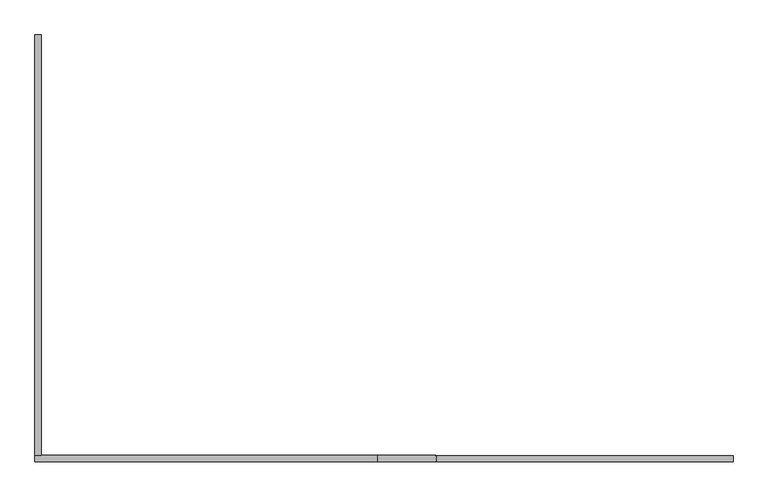
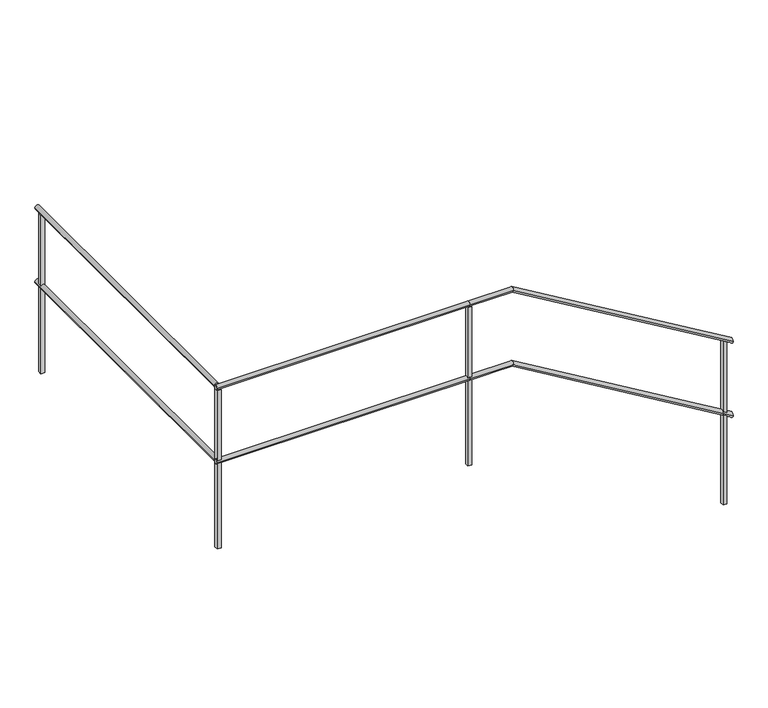
"""IFC4 building model written with IfcOpenShell, lengths in millimetres: railing geometry."""

from ifc_helpers import new_model, si_unit, frame, origin, place, context, project, spatial, polyline, circle_curve, ellipse_curve, outline, extrude, source, transform, mapped, element, save
from ifc_brep_helpers import plane_surface, cylinder_surface, advanced_brep


def railing_f3a6625a(model_context):
    return source(origin(), model_context, "Body", "SolidModel", [
        advanced_brep(
        [(26565.4, 649.5208589, 1734.9618634), (26535.4, 649.5208589, 1734.9618634), (26565.4, -1335.0791411, 1734.9618634), (26535.4, -1335.0791411, 1734.9618634)],
        [
            (0, 1, circle_curve(frame((26550.4, 649.5208589, 1734.9618634), z_axis=(0.0, 1.0, 0.0), x_axis=(-1.0, 0.0, 0.0)), 15.0)),
            (1, 0, circle_curve(frame((26550.4, 649.5208589, 1734.9618634), z_axis=(0.0, 1.0, 0.0), x_axis=(-1.0, 0.0, 0.0)), 15.0)),
            (2, 3, circle_curve(frame((26550.4, -1335.0791411, 1734.9618634), z_axis=(0.0, -1.0, 0.0), x_axis=(-1.0, 0.0, 0.0)), 15.0)),
            (3, 2, circle_curve(frame((26550.4, -1335.0791411, 1734.9618634), z_axis=(0.0, -1.0, 0.0), x_axis=(-1.0, 0.0, 0.0)), 15.0)),
            (0, 2),
            (3, 1),
        ],
        [
            plane_surface(frame((26550.4, 649.5208589, 1749.9618634), z_axis=(0.0, 1.0, 0.0), x_axis=(0.0, 0.0, -1.0))),
            plane_surface(frame((26550.4, -1335.0791411, 1749.9618634), z_axis=(0.0, -1.0, 0.0), x_axis=(0.0, 0.0, -1.0))),
            cylinder_surface(frame((26550.4, 649.5208589, 1734.9618634), z_axis=(0.0, 1.0, 0.0), x_axis=(-1.0, 0.0, 0.0)), 15.0),
        ],
        [
            (0, [[1, 2]]),
            (1, [[3, 4]]),
            (2, [[-1, 5, -4, 6]]),
            (2, [[-2, -6, -3, -5]]),
        ],
    ),
        advanced_brep(
        [(26535.4, -1335.0791411, 1734.9618634), (26535.4, -1365.0791411, 1734.9618634), (28150.0, -1335.0791411, 1734.9618634), (28150.0, -1365.0791411, 1734.9618634)],
        [
            (0, 1, circle_curve(frame((26535.4, -1350.0791411, 1734.9618634), z_axis=(-1.0, 0.0, 0.0), x_axis=(0.0, -1.0, 0.0)), 15.0)),
            (1, 0, circle_curve(frame((26535.4, -1350.0791411, 1734.9618634), z_axis=(-1.0, 0.0, 0.0), x_axis=(0.0, -1.0, 0.0)), 15.0)),
            (2, 3, circle_curve(frame((28150.0, -1350.0791411, 1734.9618634), z_axis=(1.0, 0.0, 0.0), x_axis=(0.0, -1.0, 0.0)), 15.0)),
            (3, 2, circle_curve(frame((28150.0, -1350.0791411, 1734.9618634), z_axis=(1.0, 0.0, 0.0), x_axis=(0.0, -1.0, 0.0)), 15.0)),
            (0, 2),
            (3, 1),
        ],
        [
            plane_surface(frame((26535.4, -1350.0791411, 1749.9618634), z_axis=(-1.0, 0.0, 0.0), x_axis=(0.0, 1.0, 0.0))),
            plane_surface(frame((28150.0, -1350.0791411, 1749.9618634), z_axis=(1.0, 0.0, 0.0), x_axis=(0.0, 1.0, 0.0))),
            cylinder_surface(frame((26535.4, -1350.0791411, 1734.9618634), z_axis=(-1.0, 0.0, 0.0), x_axis=(0.0, -1.0, 0.0)), 15.0),
        ],
        [
            (0, [[1, 2]]),
            (1, [[3, 4]]),
            (2, [[-1, 5, -4, 6]]),
            (2, [[-2, -6, -3, -5]]),
        ],
    ),
        advanced_brep(
        [(28150.0, -1335.0791411, 1734.9618634), (28150.0, -1365.0791411, 1734.9618634), (28425.8735614, -1335.0791411, 1734.9618634), (28425.8735614, -1365.0791411, 1734.9618634), (29830.0, -1335.0791411, 899.1723166), (29830.0, -1365.0791411, 899.1723166)],
        [
            (0, 1, circle_curve(frame((28150.0, -1350.0791411, 1734.9618634), z_axis=(-1.0, 0.0, 0.0), x_axis=(0.0, -1.0, 0.0)), 15.0)),
            (1, 0, circle_curve(frame((28150.0, -1350.0791411, 1734.9618634), z_axis=(-1.0, 0.0, 0.0), x_axis=(0.0, -1.0, 0.0)), 15.0)),
            (0, 2),
            (2, 3, ellipse_curve(frame((28425.8735614, -1350.0791411, 1734.9618634), z_axis=(-0.9641817474962141, 0.0, 0.26524245096731175), x_axis=(-0.26524245096731197, 0.0, -0.964181747496214)), 15.5572329, 15.0)),
            (3, 1),
            (3, 2, ellipse_curve(frame((28425.8735614, -1350.0791411, 1734.9618634), z_axis=(-0.9641817474962141, 0.0, 0.26524245096731175), x_axis=(-0.26524245096731197, 0.0, -0.964181747496214)), 15.5572329, 15.0)),
            (4, 5, ellipse_curve(frame((29830.0, -1350.0791411, 899.1723166), z_axis=(1.0, 0.0, 0.0), x_axis=(0.0, 0.0, 1.0)), 17.4562134, 15.0)),
            (5, 4, ellipse_curve(frame((29830.0, -1350.0791411, 899.1723166), z_axis=(1.0, 0.0, 0.0), x_axis=(0.0, 0.0, 1.0)), 17.4562134, 15.0)),
            (2, 4),
            (5, 3),
        ],
        [
            plane_surface(frame((28150.0, -1350.0791411, 1749.9618634), z_axis=(-1.0, 0.0, 0.0), x_axis=(0.0, 1.0, 0.0))),
            cylinder_surface(frame((28150.0, -1350.0791411, 1734.9618634), z_axis=(-1.0, 0.0, 0.0), x_axis=(0.0, -1.0, 0.0)), 15.0),
            plane_surface(frame((29830.0, -1350.0791411, 916.62853), z_axis=(1.0, 0.0, 0.0), x_axis=(0.0, 1.0, 0.0))),
            cylinder_surface(frame((28422.3277421, -1350.0791411, 1737.0724701), z_axis=(-0.8592928844097064, 0.0, 0.5114838597676831), x_axis=(0.0, -1.0, 0.0)), 15.0),
        ],
        [
            (0, [[1, 2]]),
            (1, [[-1, 3, 4, 5]]),
            (1, [[-2, -5, 6, -3]]),
            (2, [[7, 8]]),
            (3, [[-4, 9, -8, 10]]),
            (3, [[-6, -10, -7, -9]]),
        ],
    ),
        advanced_brep(
        [(26565.4, 649.5208589, 2234.9618634), (26535.4, 649.5208589, 2234.9618634), (26565.4, -1335.0791411, 2234.9618634), (26535.4, -1335.0791411, 2234.9618634)],
        [
            (0, 1, circle_curve(frame((26550.4, 649.5208589, 2234.9618634), z_axis=(0.0, 1.0, 0.0), x_axis=(-1.0, 0.0, 0.0)), 15.0)),
            (1, 0, circle_curve(frame((26550.4, 649.5208589, 2234.9618634), z_axis=(0.0, 1.0, 0.0), x_axis=(-1.0, 0.0, 0.0)), 15.0)),
            (2, 3, circle_curve(frame((26550.4, -1335.0791411, 2234.9618634), z_axis=(0.0, -1.0, 0.0), x_axis=(-1.0, 0.0, 0.0)), 15.0)),
            (3, 2, circle_curve(frame((26550.4, -1335.0791411, 2234.9618634), z_axis=(0.0, -1.0, 0.0), x_axis=(-1.0, 0.0, 0.0)), 15.0)),
            (0, 2),
            (3, 1),
        ],
        [
            plane_surface(frame((26550.4, 649.5208589, 2249.9618634), z_axis=(0.0, 1.0, 0.0), x_axis=(0.0, 0.0, -1.0))),
            plane_surface(frame((26550.4, -1335.0791411, 2249.9618634), z_axis=(0.0, -1.0, 0.0), x_axis=(0.0, 0.0, -1.0))),
            cylinder_surface(frame((26550.4, 649.5208589, 2234.9618634), z_axis=(0.0, 1.0, 0.0), x_axis=(-1.0, 0.0, 0.0)), 15.0),
        ],
        [
            (0, [[1, 2]]),
            (1, [[3, 4]]),
            (2, [[-1, 5, -4, 6]]),
            (2, [[-2, -6, -3, -5]]),
        ],
    ),
        advanced_brep(
        [(26535.4, -1335.0791411, 2234.9618634), (26535.4, -1365.0791411, 2234.9618634), (28150.0, -1335.0791411, 2234.9618634), (28150.0, -1365.0791411, 2234.9618634)],
        [
            (0, 1, circle_curve(frame((26535.4, -1350.0791411, 2234.9618634), z_axis=(-1.0, 0.0, 0.0), x_axis=(0.0, -1.0, 0.0)), 15.0)),
            (1, 0, circle_curve(frame((26535.4, -1350.0791411, 2234.9618634), z_axis=(-1.0, 0.0, 0.0), x_axis=(0.0, -1.0, 0.0)), 15.0)),
            (2, 3, circle_curve(frame((28150.0, -1350.0791411, 2234.9618634), z_axis=(1.0, 0.0, 0.0), x_axis=(0.0, -1.0, 0.0)), 15.0)),
            (3, 2, circle_curve(frame((28150.0, -1350.0791411, 2234.9618634), z_axis=(1.0, 0.0, 0.0), x_axis=(0.0, -1.0, 0.0)), 15.0)),
            (0, 2),
            (3, 1),
        ],
        [
            plane_surface(frame((26535.4, -1350.0791411, 2249.9618634), z_axis=(-1.0, 0.0, 0.0), x_axis=(0.0, 1.0, 0.0))),
            plane_surface(frame((28150.0, -1350.0791411, 2249.9618634), z_axis=(1.0, 0.0, 0.0), x_axis=(0.0, 1.0, 0.0))),
            cylinder_surface(frame((26535.4, -1350.0791411, 2234.9618634), z_axis=(-1.0, 0.0, 0.0), x_axis=(0.0, -1.0, 0.0)), 15.0),
        ],
        [
            (0, [[1, 2]]),
            (1, [[3, 4]]),
            (2, [[-1, 5, -4, 6]]),
            (2, [[-2, -6, -3, -5]]),
        ],
    ),
        advanced_brep(
        [(28150.0, -1335.0791411, 2234.9618634), (28150.0, -1365.0791411, 2234.9618634), (28425.8735614, -1335.0791411, 2234.9618634), (28425.8735614, -1365.0791411, 2234.9618634), (29830.0, -1335.0791411, 1399.1723166), (29830.0, -1365.0791411, 1399.1723166)],
        [
            (0, 1, circle_curve(frame((28150.0, -1350.0791411, 2234.9618634), z_axis=(-1.0, 0.0, 0.0), x_axis=(0.0, -1.0, 0.0)), 15.0)),
            (1, 0, circle_curve(frame((28150.0, -1350.0791411, 2234.9618634), z_axis=(-1.0, 0.0, 0.0), x_axis=(0.0, -1.0, 0.0)), 15.0)),
            (0, 2),
            (2, 3, ellipse_curve(frame((28425.8735614, -1350.0791411, 2234.9618634), z_axis=(-0.9641817474962141, 0.0, 0.26524245096731175), x_axis=(-0.26524245096731197, 0.0, -0.964181747496214)), 15.5572329, 15.0)),
            (3, 1),
            (3, 2, ellipse_curve(frame((28425.8735614, -1350.0791411, 2234.9618634), z_axis=(-0.9641817474962141, 0.0, 0.26524245096731175), x_axis=(-0.26524245096731197, 0.0, -0.964181747496214)), 15.5572329, 15.0)),
            (4, 5, ellipse_curve(frame((29830.0, -1350.0791411, 1399.1723166), z_axis=(1.0, 0.0, 0.0), x_axis=(0.0, 0.0, 1.0)), 17.4562134, 15.0)),
            (5, 4, ellipse_curve(frame((29830.0, -1350.0791411, 1399.1723166), z_axis=(1.0, 0.0, 0.0), x_axis=(0.0, 0.0, 1.0)), 17.4562134, 15.0)),
            (2, 4),
            (5, 3),
        ],
        [
            plane_surface(frame((28150.0, -1350.0791411, 2249.9618634), z_axis=(-1.0, 0.0, 0.0), x_axis=(0.0, 1.0, 0.0))),
            cylinder_surface(frame((28150.0, -1350.0791411, 2234.9618634), z_axis=(-1.0, 0.0, 0.0), x_axis=(0.0, -1.0, 0.0)), 15.0),
            plane_surface(frame((29830.0, -1350.0791411, 1416.62853), z_axis=(1.0, 0.0, 0.0), x_axis=(0.0, 1.0, 0.0))),
            cylinder_surface(frame((28422.3277421, -1350.0791411, 2237.0724701), z_axis=(-0.8592928844097064, 0.0, 0.5114838597676831), x_axis=(0.0, -1.0, 0.0)), 15.0),
        ],
        [
            (0, [[1, 2]]),
            (1, [[-1, 3, 4, 5]]),
            (1, [[-2, -5, 6, -3]]),
            (2, [[7, 8]]),
            (3, [[-4, 9, -8, 10]]),
            (3, [[-6, -10, -7, -9]]),
        ],
    ),
        extrude(outline(polyline([(28137.5, -1362.5791411), (28137.5, -1337.5791411), (28162.5, -1337.5791411), (28162.5, -1362.5791411), (28137.5, -1362.5791411)])), frame((0.0, 0.0, 1149.9618634), z_axis=(0.0, 0.0, 1.0), x_axis=(1.0, 0.0, 0.0)), (0.0, 0.0, 1.0), 1070.0),
        extrude(outline(polyline([(26537.9, -1337.5791411), (26562.9, -1337.5791411), (26562.9, -1362.5791411), (26537.9, -1362.5791411), (26537.9, -1337.5791411)])), frame((0.0, 0.0, 1149.9618634), z_axis=(0.0, 0.0, 1.0), x_axis=(1.0, 0.0, 0.0)), (0.0, 0.0, 1.0), 1070.0),
        extrude(outline(polyline([(1423.830911, 29767.5), (316.62853, 29767.5), (316.62853, 29792.5), (1408.9499586, 29792.5), (1423.830911, 29767.5)])), frame((0.0, -1362.5791411, 0.0), z_axis=(0.0, 1.0, 0.0), x_axis=(0.0, 0.0, 1.0)), (0.0, 0.0, 1.0), 25.0),
        extrude(outline(polyline([(26537.9, 612.0208589), (26562.9, 612.0208589), (26562.9, 587.0208589), (26537.9, 587.0208589), (26537.9, 612.0208589)])), frame((0.0, 0.0, 1149.9618634), z_axis=(0.0, 0.0, 1.0), x_axis=(1.0, 0.0, 0.0)), (0.0, 0.0, 1.0), 1070.0),
    ])


if __name__ == "__main__":
    model = new_model("IFC4")
    model_context = context("Model", 3, world=origin())
    ifc_project = project(units=[si_unit("LENGTHUNIT", "METRE", prefix="MILLI")], contexts=[model_context])
    site = spatial("IfcSite", under=ifc_project)
    building = spatial("IfcBuilding", under=site)
    placement = place(None, origin())
    railing_shape = railing_f3a6625a(model_context)
    element("IfcRailing", 1, at=placement, inside=building, context=model_context, shape_type="MappedRepresentation", body=[
        mapped(railing_shape, transform((0.0, 0.0, 0.0), x_axis=(1.0, 0.0, 0.0), y_axis=(0.0, 1.0, 0.0), z_axis=(0.0, 0.0, 1.0))),
    ])
    save(model, "model.ifc")
